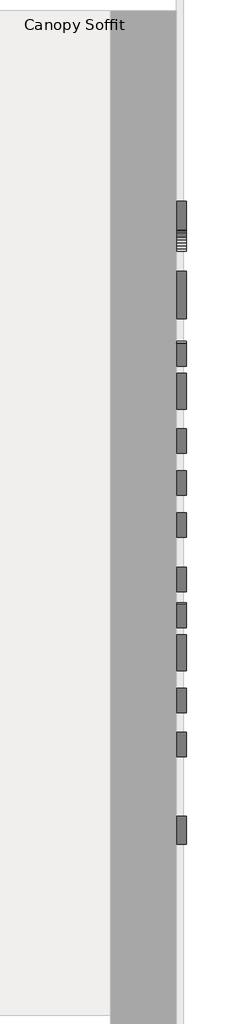
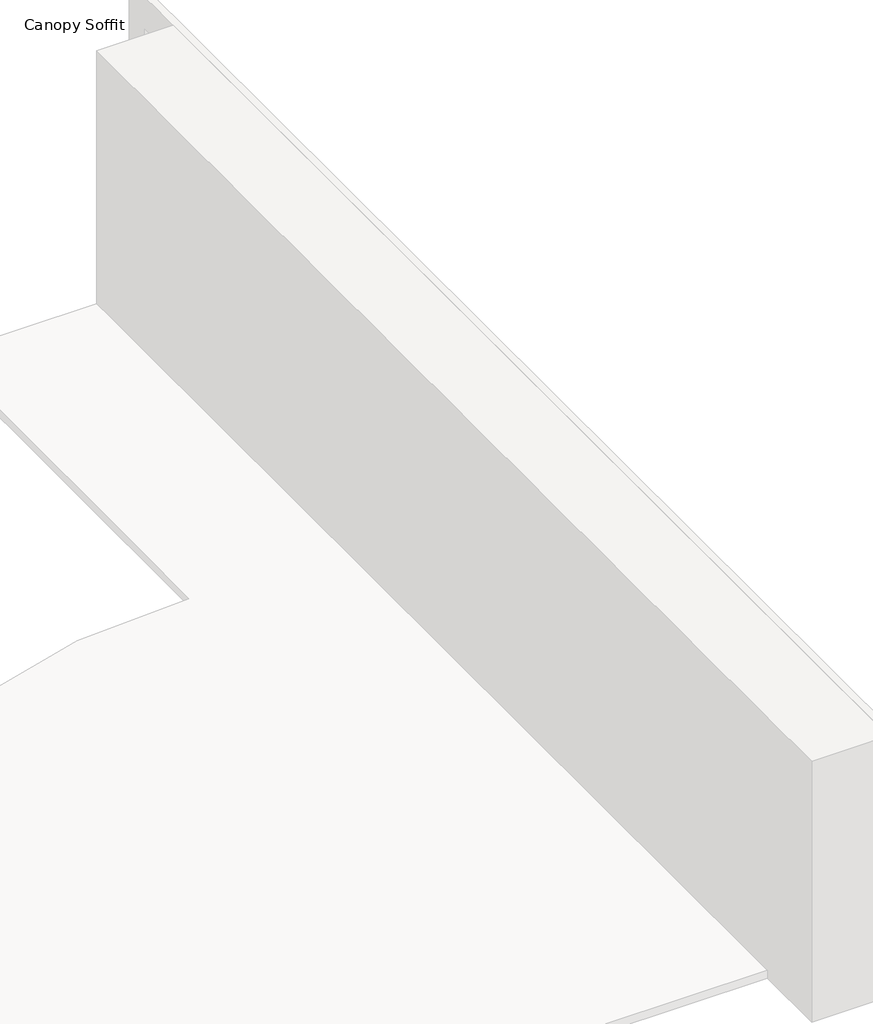
# One storey, part 2 of 2: 1 proxy.
"""IFC4 building model written with IfcOpenShell, lengths in millimetres."""

from ifc_helpers import new_model, si_unit, frame, origin, place, context, project, spatial, polyline, outline, extrude, element, save

model = new_model("IFC4")

# Units and contexts
model_context = context("Model", 3, world=origin())
ifc_project = project(units=[si_unit("LENGTHUNIT", "METRE", prefix="MILLI")], contexts=[model_context])

# Site, building, storey
site = spatial("IfcSite", under=ifc_project)
building = spatial("IfcBuilding", under=site)
storey = spatial("IfcBuildingStorey", under=building, Name="Canopy Soffit", Elevation=4572.0)

# Proxy
placement = place(None, origin())
element("IfcBuildingElementProxy", 1, Name="big", ObjectType="big", at=placement, inside=storey, context=model_context, shape_type="SweptSolid", body=[
    extrude(outline(polyline([(-13815.1592302, 7081.4539876), (-13114.5433623, 7081.4539876), (-13059.1440865, 7079.584566), (-13007.3325232, 7073.976301), (-12959.1086725, 7064.6291927), (-12914.4725344, 7051.5432411), (-12873.4241089, 7034.7184463), (-12835.9633959, 7014.1548081), (-12802.0903954, 6989.8523266), (-12771.8051075, 6961.8110018), (-12745.0943904, 6930.3265242), (-12721.9451022, 6895.6945846), (-12702.357243, 6857.9151828), (-12686.3308127, 6816.988319), (-12673.8658114, 6772.913993), (-12664.962239, 6725.6922049), (-12659.6200956, 6675.3229547), (-12657.8393811, 6621.8062423), (-12659.76137, 6566.5876663), (-12665.5273366, 6514.4771271), (-12675.137281, 6465.4746245), (-12688.5912031, 6419.5801586), (-12705.8891029, 6376.7937294), (-12727.0309805, 6337.115337), (-12752.0168358, 6300.5449812), (-12780.8466689, 6267.0826621), (-12813.6190432, 6237.1686302), (-12850.4325223, 6211.2431359), (-12891.2871063, 6189.3061792), (-12936.182795, 6171.35776), (-12985.1195886, 6157.3978785), (-13038.097487, 6147.4265345), (-13095.1164901, 6141.4437281), (-13156.1765981, 6139.4494593), (-13384.5285887, 6139.4494593), (-13384.5285887, 5708.8188178), (-13815.1592302, 5708.8188178), (-13815.1592302, 7081.4539876)]), holes=[polyline([(-13384.5285887, 6462.4224404), (-13289.9075981, 6462.4224404), (-13238.3391582, 6464.9982341), (-13195.0763387, 6472.725615), (-13160.1191394, 6485.6045831), (-13133.4675604, 6503.6351386), (-13113.7811376, 6525.6870861), (-13099.7194071, 6550.6302305), (-13091.2823687, 6578.4645719), (-13088.4700226, 6609.1901103), (-13090.9143982, 6639.1402821), (-13098.247525, 6666.7512128), (-13110.4694029, 6692.0229024), (-13127.5800321, 6714.9553508), (-13151.4455486, 6733.9978252), (-13183.9320887, 6747.5995926), (-13225.0396524, 6755.760653), (-13274.7682396, 6758.4810065), (-13384.5285887, 6758.4810065), (-13384.5285887, 6462.4224404)])]), frame((21878.1272279, 0.0, 0.0), z_axis=(1.0, 0.0, 0.0), x_axis=(0.0, 1.0, 0.0)), (0.0, 0.0, 1.0), 152.4),
    extrude(outline(polyline([(-12469.4384755, 7081.4539876), (-12092.6366641, 7081.4539876), (-12092.6366641, 6582.2756952), (-12053.776349, 6619.5721356), (-12014.9948847, 6651.1387494), (-11976.2922712, 6676.9755365), (-11937.6685085, 6697.082497), (-11897.3363113, 6712.1692883), (-11853.5083941, 6722.9455678), (-11806.184757, 6729.4113355), (-11755.3654, 6731.5665914), (-11681.4953183, 6725.6264959), (-11647.6650288, 6718.2013765), (-11615.9045733, 6707.8062093), (-11586.2139521, 6694.4409944), (-11558.593165, 6678.1057317), (-11533.0422121, 6658.8004213), (-11509.5610934, 6636.5250631), (-11488.5177793, 6611.1745227), (-11470.2802405, 6582.6436657), (-11454.8484769, 6550.932492), (-11442.2224884, 6516.0410018), (-11432.4022752, 6477.9691949), (-11425.3878372, 6436.7170713), (-11419.7762868, 6344.6718744), (-11419.7762868, 5708.8188178), (-11796.5780981, 5708.8188178), (-11796.5780981, 6262.2464782), (-11798.8122048, 6306.1006789), (-11805.514525, 6343.0422907), (-11816.6850586, 6373.0713134), (-11832.3238057, 6396.187747), (-11851.9839448, 6413.3903688), (-11875.2186547, 6425.6779558), (-11902.0279354, 6433.050508), (-11932.4117868, 6435.5080253), (-11966.4622016, 6432.1962907), (-11997.1220309, 6422.2610867), (-12024.3912747, 6405.7024133), (-12048.269933, 6382.5202706), (-12067.6803779, 6350.743388), (-12081.5449814, 6308.4004947), (-12089.8637434, 6255.4915908), (-12092.6366641, 6192.0166763), (-12092.6366641, 5708.8188178), (-12469.4384755, 5708.8188178), (-12469.4384755, 7081.4539876)])), frame((21878.1272279, 0.0, 0.0), z_axis=(1.0, 0.0, 0.0), x_axis=(0.0, 1.0, 0.0)), (0.0, 0.0, 1.0), 152.4),
    extrude(outline(polyline([(-10827.6591547, 6354.7647801), (-11204.460966, 6381.6791952), (-11193.2378652, 6433.4184785), (-11179.7543741, 6479.2965171), (-11164.0104926, 6519.313311), (-11146.0062207, 6553.4688603), (-11124.7690651, 6583.6818682), (-11099.3265321, 6611.8710383), (-11069.6786217, 6638.0363706), (-11035.825334, 6662.177865), (-11007.7412983, 6677.6720522), (-10974.794795, 6691.3526704), (-10894.3143858, 6713.2731999), (-10800.3767691, 6726.9932435), (-10698.9746075, 6731.5665914), (-10546.950216, 6726.7304074), (-10483.3964507, 6720.6851775), (-10428.1483057, 6712.2218555), (-10379.181943, 6699.9474104), (-10334.473525, 6682.4688107), (-10294.0230515, 6659.7860566), (-10257.8305226, 6631.899148), (-10235.1346267, 6608.4541692), (-10214.9882408, 6580.5935442), (-10197.3913649, 6548.317273), (-10182.3439991, 6511.6253555), (-10161.6850828, 6435.6131598), (-10156.5203537, 6398.9475259), (-10154.7987774, 6363.1755348), (-10154.7987774, 5921.6109121), (-10152.5909542, 5858.6353862), (-10145.9674849, 5811.0094876), (-10131.7743363, 5765.4862777), (-10106.8574755, 5708.8188178), (-10468.0993906, 5708.8188178), (-10496.4856877, 5783.8848036), (-10509.7326264, 5864.8383178), (-10545.8463045, 5822.4428573), (-10581.8548481, 5786.5131645), (-10617.7582573, 5757.0492394), (-10653.5565321, 5734.0510819), (-10704.5204489, 5711.2369098), (-10759.4269071, 5694.9410725), (-10818.2759065, 5685.1635702), (-10881.0674472, 5681.9044027), (-10961.8895433, 5686.9508555), (-11032.3558976, 5702.090214), (-11063.7056717, 5713.4447329), (-11092.4665103, 5727.3224782), (-11118.6384134, 5743.7234499), (-11142.2213811, 5762.647648), (-11181.2262561, 5805.3847954), (-11209.0868811, 5852.8529923), (-11225.8032561, 5905.0522388), (-11231.3753811, 5961.9825348), (-11227.353989, 6015.0228567), (-11215.2898127, 6063.1218603), (-11195.1828522, 6106.2795454), (-11167.0331075, 6144.4959121), (-11128.264785, 6177.9549457), (-11075.8815533, 6206.8406315), (-11009.8834124, 6231.1529693), (-10930.2703623, 6250.8919593), (-10759.6897432, 6287.0056374), (-10661.7570179, 6310.3980489), (-10598.4135215, 6330.0056209), (-10531.6005887, 6354.7647801), (-10533.2301724, 6382.3888526), (-10538.1189236, 6405.5447117), (-10546.2668422, 6424.2323573), (-10557.6739283, 6438.4517895), (-10573.1549737, 6448.9389493), (-10593.5247703, 6456.4297777), (-10618.783318, 6460.9242748), (-10648.930617, 6462.4224404), (-10688.3297461, 6460.7140059), (-10722.4195863, 6455.5887022), (-10751.2001376, 6447.0465295), (-10774.6714, 6435.0874876), (-10790.2838634, 6422.0245342), (-10804.3193104, 6404.2830985), (-10816.7777408, 6381.8631804), (-10827.6591547, 6354.7647801)]), holes=[polyline([(-10531.6005887, 6166.3638744), (-10607.1922467, 6146.1780631), (-10685.9379377, 6128.5154782), (-10775.3022066, 6105.1756338), (-10805.0026842, 6093.6634133), (-10824.7153906, 6082.2563272), (-10837.778344, 6070.0870165), (-10847.109025, 6057.1291975), (-10852.7074336, 6043.3828703), (-10854.5735698, 6028.8480348), (-10852.7205754, 6012.4076377), (-10847.1615922, 5997.5705407), (-10837.8966202, 5984.3367438), (-10824.9256594, 5972.706247), (-10808.3801279, 5963.2310062), (-10788.3914436, 5956.462977), (-10738.084617, 5951.0485536), (-10680.1029766, 5956.9360819), (-10626.4318481, 5974.5986669), (-10582.3805203, 6000.7245737), (-10565.953265, 6015.7193723), (-10553.2582821, 6032.0020678), (-10543.7830412, 6050.2034667), (-10537.015012, 6070.9543756), (-10531.6005887, 6120.1047235), (-10531.6005887, 6166.3638744)])]), frame((21878.1272279, 0.0, 0.0), z_axis=(1.0, 0.0, 0.0), x_axis=(0.0, 1.0, 0.0)), (0.0, 0.0, 1.0), 152.4),
    extrude(outline(polyline([(-9939.4834566, 6704.6521763), (-9588.3344472, 6704.6521763), (-9588.3344472, 6544.4272989), (-9562.2479657, 6593.6696394), (-9535.714663, 6634.5800761), (-9508.7345389, 6667.1586088), (-9481.3075934, 6691.4052376), (-9452.0407953, 6708.9758299), (-9419.5411134, 6721.5262529), (-9383.8085477, 6729.0565068), (-9344.8430981, 6731.5665914), (-9301.3700097, 6728.0445878), (-9255.899367, 6717.4785772), (-9208.43117, 6699.8685595), (-9158.9654189, 6675.2145348), (-9277.9775981, 6407.331997), (-9338.9555698, 6428.4640183), (-9385.6352585, 6435.5080253), (-9421.3546824, 6431.6180513), (-9452.8161618, 6419.9481291), (-9480.0196966, 6400.4982588), (-9502.9652868, 6373.2684404), (-9516.9613083, 6348.9101063), (-9529.0911936, 6319.7812972), (-9547.7525557, 6247.2122541), (-9558.9493729, 6155.5613113), (-9562.6816453, 6044.8284687), (-9562.6816453, 5708.8188178), (-9939.4834566, 5708.8188178), (-9939.4834566, 6704.6521763)])), frame((21878.1272279, 0.0, 0.0), z_axis=(1.0, 0.0, 0.0), x_axis=(0.0, 1.0, 0.0)), (0.0, 0.0, 1.0), 152.4),
    extrude(outline(polyline([(-9105.1365887, 6704.6521763), (-8753.9875792, 6704.6521763), (-8753.9875792, 6564.1925725), (-8715.8500633, 6606.3251969), (-8677.5548457, 6641.8869192), (-8639.1019265, 6670.8777394), (-8600.4913057, 6693.2976574), (-8559.7779961, 6710.040316), (-8515.0170108, 6721.9993579), (-8466.2083499, 6729.174783), (-8413.3520132, 6731.5665914), (-8357.5519124, 6728.9382305), (-8307.9021759, 6721.053148), (-8264.4028039, 6707.9113437), (-8227.0537962, 6689.5128178), (-8194.3307037, 6665.9101374), (-8164.7090769, 6637.1558697), (-8138.1889159, 6603.2500147), (-8114.7702207, 6564.1925725), (-8071.3759831, 6608.8878488), (-8029.9267325, 6645.8294605), (-7990.422469, 6675.0174077), (-7952.8631924, 6696.4516904), (-7914.1474371, 6711.8144596), (-7871.1737373, 6722.7878661), (-7823.9420928, 6729.3719101), (-7772.4525038, 6731.5665914), (-7697.715063, 6725.5870705), (-7663.5890829, 6718.1126693), (-7631.6249295, 6707.6485077), (-7601.8226029, 6694.1945856), (-7574.1821031, 6677.750903), (-7548.7034301, 6658.31746), (-7525.386584, 6635.8942565), (-7504.540397, 6610.2973073), (-7486.4737016, 6581.3426271), (-7471.1864978, 6549.0302159), (-7458.6787856, 6513.3600737), (-7448.950565, 6474.3322005), (-7442.001836, 6431.9465964), (-7436.4428528, 6337.1021952), (-7436.4428528, 5708.8188178), (-7813.2446641, 5708.8188178), (-7813.2446641, 6282.0117518), (-7814.8742479, 6313.8937689), (-7819.7629991, 6341.4127069), (-7827.9109177, 6364.568566), (-7839.3180038, 6383.3613461), (-7859.4249643, 6406.1755183), (-7881.8974495, 6422.4713555), (-7906.7354595, 6432.2488579), (-7933.9389943, 6435.5080253), (-7965.7421606, 6432.4328432), (-7994.2861594, 6423.2072966), (-8019.5709908, 6407.8313856), (-8041.5966547, 6386.3051103), (-8059.4432249, 6357.9713803), (-8072.190775, 6322.1731055), (-8079.8393051, 6278.910286), (-8082.3888151, 6228.1829216), (-8082.3888151, 5708.8188178), (-8459.1906264, 5708.8188178), (-8459.1906264, 6261.8259404), (-8461.0830462, 6317.2317871), (-8466.7603057, 6351.4004782), (-8483.3715462, 6385.5691692), (-8508.8140792, 6412.3784499), (-8541.1954849, 6429.7256315), (-8578.6233434, 6435.5080253), (-8609.9534047, 6432.3802759), (-8638.3397019, 6422.9970277), (-8663.7822349, 6407.3582807), (-8686.2810038, 6385.4640348), (-8704.6795297, 6356.4206474), (-8717.821334, 6319.3344758), (-8725.7064165, 6274.20552), (-8728.3347774, 6221.0337801), (-8728.3347774, 5708.8188178), (-9105.1365887, 5708.8188178), (-9105.1365887, 6704.6521763)])), frame((21878.1272279, 0.0, 0.0), z_axis=(1.0, 0.0, 0.0), x_axis=(0.0, 1.0, 0.0)), (0.0, 0.0, 1.0), 152.4),
    extrude(outline(polyline([(-6817.4113057, 6354.7647801), (-7194.213117, 6381.6791952), (-7182.9900162, 6433.4184785), (-7169.506525, 6479.2965171), (-7153.7626435, 6519.313311), (-7135.7583717, 6553.4688603), (-7114.521216, 6583.6818682), (-7089.078683, 6611.8710383), (-7059.4307726, 6638.0363706), (-7025.5774849, 6662.177865), (-6997.4934492, 6677.6720522), (-6964.546946, 6691.3526704), (-6884.0665368, 6713.2731999), (-6790.12892, 6726.9932435), (-6688.7267585, 6731.5665914), (-6536.702367, 6726.7304074), (-6473.1486016, 6720.6851775), (-6417.9004566, 6712.2218555), (-6368.934094, 6699.9474104), (-6324.2256759, 6682.4688107), (-6283.7752025, 6659.7860566), (-6247.5826736, 6631.899148), (-6224.8867776, 6608.4541692), (-6204.7403917, 6580.5935442), (-6187.1435159, 6548.317273), (-6172.09615, 6511.6253555), (-6151.4372337, 6435.6131598), (-6146.2725047, 6398.9475259), (-6144.5509283, 6363.1755348), (-6144.5509283, 5921.6109121), (-6142.3431052, 5858.6353862), (-6135.7196358, 5811.0094876), (-6121.5264873, 5765.4862777), (-6096.6096264, 5708.8188178), (-6457.8515415, 5708.8188178), (-6486.2378387, 5783.8848036), (-6499.4847774, 5864.8383178), (-6535.5984554, 5822.4428573), (-6571.6069991, 5786.5131645), (-6607.5104082, 5757.0492394), (-6643.308683, 5734.0510819), (-6694.2725999, 5711.2369098), (-6749.179058, 5694.9410725), (-6808.0280574, 5685.1635702), (-6870.8195981, 5681.9044027), (-6951.6416942, 5686.9508555), (-7022.1080486, 5702.090214), (-7053.4578226, 5713.4447329), (-7082.2186612, 5727.3224782), (-7108.3905644, 5743.7234499), (-7131.9735321, 5762.647648), (-7170.9784071, 5805.3847954), (-7198.8390321, 5852.8529923), (-7215.5554071, 5905.0522388), (-7221.1275321, 5961.9825348), (-7217.10614, 6015.0228567), (-7205.0419637, 6063.1218603), (-7184.9350032, 6106.2795454), (-7156.7852585, 6144.4959121), (-7118.016936, 6177.9549457), (-7065.6337042, 6206.8406315), (-6999.6355633, 6231.1529693), (-6920.0225132, 6250.8919593), (-6749.4418941, 6287.0056374), (-6651.5091689, 6310.3980489), (-6588.1656724, 6330.0056209), (-6521.3527396, 6354.7647801), (-6522.9823233, 6382.3888526), (-6527.8710745, 6405.5447117), (-6536.0189932, 6424.2323573), (-6547.4260792, 6438.4517895), (-6562.9071246, 6448.9389493), (-6583.2769212, 6456.4297777), (-6608.535469, 6460.9242748), (-6638.6827679, 6462.4224404), (-6678.081897, 6460.7140059), (-6712.1717373, 6455.5887022), (-6740.9522886, 6447.0465295), (-6764.4235509, 6435.0874876), (-6780.0360144, 6422.0245342), (-6794.0714613, 6404.2830985), (-6806.5298917, 6381.8631804), (-6817.4113057, 6354.7647801)]), holes=[polyline([(-6521.3527396, 6166.3638744), (-6596.9443976, 6146.1780631), (-6675.6900887, 6128.5154782), (-6765.0543575, 6105.1756338), (-6794.7548351, 6093.6634133), (-6814.4675415, 6082.2563272), (-6827.5304949, 6070.0870165), (-6836.8611759, 6057.1291975), (-6842.4595845, 6043.3828703), (-6844.3257207, 6028.8480348), (-6842.4727264, 6012.4076377), (-6836.9137432, 5997.5705407), (-6827.6487712, 5984.3367438), (-6814.6778104, 5972.706247), (-6798.1322788, 5963.2310062), (-6778.1435946, 5956.462977), (-6727.8367679, 5951.0485536), (-6669.8551276, 5956.9360819), (-6616.1839991, 5974.5986669), (-6572.1326712, 6000.7245737), (-6555.7054159, 6015.7193723), (-6543.010433, 6032.0020678), (-6533.5351922, 6050.2034667), (-6526.767163, 6070.9543756), (-6521.3527396, 6120.1047235), (-6521.3527396, 6166.3638744)])]), frame((21878.1272279, 0.0, 0.0), z_axis=(1.0, 0.0, 0.0), x_axis=(0.0, 1.0, 0.0)), (0.0, 0.0, 1.0), 152.4),
    extrude(outline(polyline([(-5202.5464, 6085.6206291), (-4825.7445887, 6058.706214), (-4842.8289342, 6003.0375312), (-4864.6443292, 5951.2588225), (-4891.1907738, 5903.3700878), (-4922.4682679, 5859.3713272), (-4958.4373861, 5819.6567948), (-4999.0587031, 5784.6207447), (-5044.3322187, 5754.2631769), (-5094.257933, 5728.5840914), (-5150.044892, 5708.1617276), (-5212.9021417, 5693.5743249), (-5282.8296821, 5684.8218832), (-5359.8275132, 5681.9044027), (-5434.3678269, 5683.7705389), (-5502.3898057, 5689.3689475), (-5563.8934495, 5698.6996285), (-5618.8787585, 5711.7625819), (-5668.8044728, 5728.9783455), (-5715.1293328, 5750.7674569), (-5757.8533384, 5777.1299163), (-5796.9764896, 5808.0657235), (-5832.2753758, 5842.7469449), (-5863.5265863, 5880.3456468), (-5890.7301211, 5920.8618293), (-5913.8859802, 5964.2954923), (-5932.3764988, 6012.854459), (-5945.584012, 6068.7465525), (-5953.50852, 6131.9717727), (-5956.1500226, 6202.5301197), (-5952.9434224, 6276.6761792), (-5943.3236217, 6344.3564711), (-5927.2906205, 6405.5709953), (-5904.8444189, 6460.3197518), (-5884.4089133, 6497.1825127), (-5860.5302549, 6532.0740029), (-5833.2084439, 6564.9942226), (-5802.4434802, 6595.9431716), (-5769.7335294, 6624.0009236), (-5736.5767573, 6648.2475525), (-5702.9731639, 6668.6830581), (-5668.9227491, 6685.3074404), (-5610.8096907, 6705.545819), (-5544.9692514, 6720.0018036), (-5471.4014312, 6728.6753944), (-5390.1062302, 6731.5665914), (-5278.3614687, 6725.9944664), (-5227.7819496, 6719.0293101), (-5180.7310049, 6709.2780914), (-5137.2086347, 6696.7408101), (-5097.214839, 6681.4174664), (-5060.7496176, 6663.3080601), (-5027.8129707, 6642.4125914), (-4997.8003753, 6618.8361946), (-4970.1073083, 6592.6840041), (-4944.7337698, 6563.95602), (-4921.6797597, 6532.6522423), (-4900.945278, 6498.772671), (-4882.5303248, 6462.317306), (-4852.6590038, 6381.6791952), (-5229.4608151, 6354.7647801), (-5238.5549436, 6379.8262008), (-5250.6979707, 6401.6021704), (-5265.8898965, 6420.092689), (-5284.1307207, 6435.2977565), (-5305.6044289, 6447.1648057), (-5330.4950061, 6455.6412694), (-5358.8024525, 6460.7271477), (-5390.5267679, 6462.4224404), (-5430.7669725, 6458.2827721), (-5466.9595014, 6445.8637671), (-5499.1043546, 6425.1654254), (-5527.2015321, 6396.187747), (-5550.0157042, 6358.799314), (-5566.3115415, 6312.8687081), (-5576.0890439, 6258.3959295), (-5579.3482113, 6195.3809782), (-5575.9970512, 6139.0552052), (-5565.943571, 6089.9311409), (-5549.1877706, 6048.0087854), (-5525.72965, 6013.2881386), (-5497.0936585, 5986.0583202), (-5464.8042455, 5966.6084499), (-5428.8614109, 5954.9385277), (-5389.2651547, 5951.0485536), (-5355.9638228, 5953.1118169), (-5325.4485533, 5959.3016067), (-5297.7193463, 5969.617923), (-5272.7762019, 5984.0607659), (-5250.7242544, 6002.787837), (-5231.6686382, 6025.9568378), (-5215.6093534, 6053.5677686), (-5202.5464, 6085.6206291)])), frame((21878.1272279, 0.0, 0.0), z_axis=(1.0, 0.0, 0.0), x_axis=(0.0, 1.0, 0.0)), (0.0, 0.0, 1.0), 152.4),
    extrude(outline(polyline([(-4771.9157585, 6704.6521763), (-4365.6763057, 6704.6521763), (-4166.3414189, 6041.8847046), (-3985.0896547, 6704.6521763), (-3614.5959094, 6704.6521763), (-3998.9674, 5638.1684782), (-4032.5841353, 5555.269977), (-4066.568841, 5486.9851621), (-4100.9215173, 5433.3140336), (-4135.6421641, 5394.2565914), (-4161.8534927, 5373.3611226), (-4191.2845633, 5355.2517164), (-4223.935376, 5339.9283726), (-4259.8059307, 5327.3910914), (-4298.8962274, 5317.6398726), (-4341.2062662, 5310.6747164), (-4435.4855698, 5305.1025914), (-4539.6737939, 5310.8849853), (-4688.2287491, 5328.2321669), (-4718.0869283, 5599.0584687), (-4675.744035, 5588.2033384), (-4631.1407514, 5580.4496739), (-4584.2770775, 5575.7974752), (-4535.1530132, 5574.2467423), (-4503.1132945, 5575.9683187), (-4474.2801759, 5581.1330478), (-4448.6536577, 5589.7409295), (-4426.2337396, 5601.791964), (-4406.2056299, 5618.2586447), (-4387.7545368, 5640.1134652), (-4370.8804601, 5667.3564254), (-4355.5834, 5699.9875253), (-4771.9157585, 6704.6521763)])), frame((21878.1272279, 0.0, 0.0), z_axis=(1.0, 0.0, 0.0), x_axis=(0.0, 1.0, 0.0)), (0.0, 0.0, 1.0), 152.4),
])

save(model, "model.ifc")

# Revit data of these elements
# Element 1 (IfcBuildingElementProxy, "big")
#   Phase Created = New Construction
#   Materials on its faces: "Paint - Red"
# Materials
#   "Paint - Red": class "Paint", colour RGB 204 0 0, transparency 0, Cost = 0
